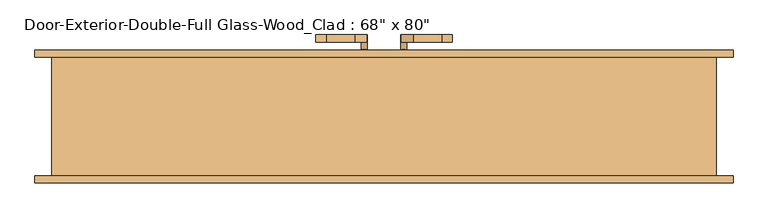
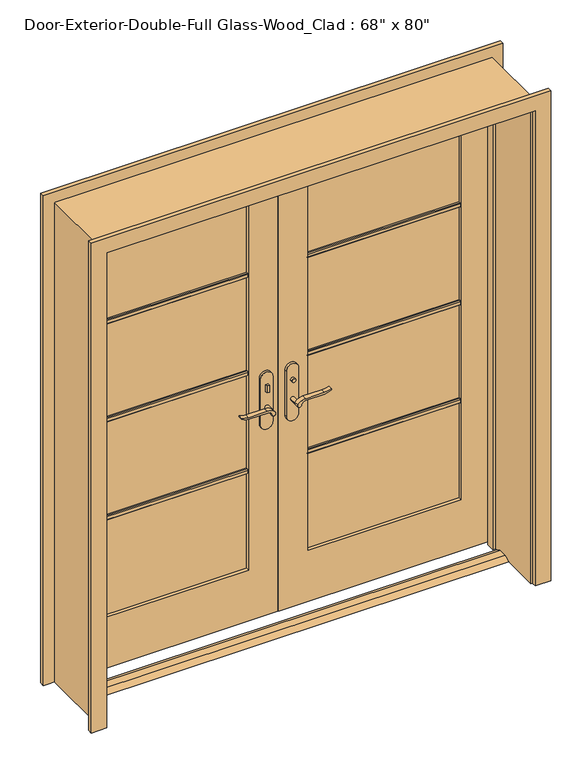
"""IFC4 building model written with IfcOpenShell, lengths in millimetres: door geometry."""

import ifcopenshell
import ifcopenshell.guid

model = None  # the IFC model being written
_history = None  # IfcOwnerHistory: only IFC2X3 demands one
_inside = {}  # id of a spatial element -> (the spatial element, [elements in it])
_under = {}  # id of a project, library or spatial element -> (it, [spatial elements below it])
_declared = {}  # id of a project -> (the project, [libraries it declares])
_typed = {}  # id of a type object -> (the type object, [elements of that type])
_made_of = {}  # id of a material, layer set ... -> (it, [elements and type objects made of it])


def new_model(schema):
    """Start an empty IFC model of exactly this schema.

    Asked for "IFC4X3", IfcOpenShell would pick the latest addendum, in which some entities
    have other attributes; the version numbers below select the first issue.
    IFC2X3 requires an IfcOwnerHistory on every rooted entity: one is made here for all.
    """
    global model, _history
    if schema == "IFC4X3":
        model = ifcopenshell.file(schema_version=(4, 3, 0, 0))
    else:
        model = ifcopenshell.file(schema=schema)
    _inside.clear()
    _under.clear()
    _declared.clear()
    _typed.clear()
    _made_of.clear()
    _history = None
    if model.schema == "IFC2X3":
        org = make("IfcOrganization", Name="unknown")
        user = make(
            "IfcPersonAndOrganization",
            ThePerson=make("IfcPerson", FamilyName="unknown"),
            TheOrganization=org,
        )
        app = make(
            "IfcApplication",
            ApplicationDeveloper=org,
            Version="unknown",
            ApplicationFullName="unknown",
            ApplicationIdentifier="unknown",
        )
        _history = make(
            "IfcOwnerHistory",
            OwningUser=user,
            OwningApplication=app,
            ChangeAction="ADDED",
            CreationDate=0,
        )
    return model


def make(cls, **values):
    """One entity of the class cls with the attributes given. An attribute that is None is left unset."""
    return model.create_entity(
        cls, **{name: value for name, value in values.items() if value is not None}
    )


def rooted(cls, **values):
    """An entity with a GlobalId (a new one), such as an element, a storey or a relation."""
    return make(cls, GlobalId=ifcopenshell.guid.new(), OwnerHistory=_history, **values)


def si_unit(unit_type, name, prefix=None):
    """IfcSIUnit, for example si_unit("LENGTHUNIT", "METRE", prefix="MILLI")."""
    return make("IfcSIUnit", UnitType=unit_type, Prefix=prefix, Name=name)


def assignment(units):
    """IfcUnitAssignment: the units of a project."""
    return None if units is None else make("IfcUnitAssignment", Units=units)


def point(xyz):
    """IfcCartesianPoint."""
    return None if xyz is None else make("IfcCartesianPoint", Coordinates=xyz)


def direction(xyz):
    """IfcDirection."""
    return None if xyz is None else make("IfcDirection", DirectionRatios=xyz)


def frame(location, z_axis=None, x_axis=None):
    """IfcAxis2Placement3D, a coordinate frame: its origin and axes. An axis left out is left unset."""
    return make(
        "IfcAxis2Placement3D",
        Location=point(location),
        Axis=direction(z_axis),
        RefDirection=direction(x_axis),
    )


def frame_2d(location, x_axis=None):
    """IfcAxis2Placement2D, a coordinate frame in the plane: its origin and x axis."""
    return make(
        "IfcAxis2Placement2D", Location=point(location), RefDirection=direction(x_axis)
    )


def origin():
    """The frame at (0, 0, 0) with its axes left unset."""
    return frame((0.0, 0.0, 0.0))


def place(relative_to, where):
    """IfcLocalPlacement: puts the frame where relative to a parent placement (None: the world)."""
    return make(
        "IfcLocalPlacement", PlacementRelTo=relative_to, RelativePlacement=where
    )


def context(
    kind, dimensions, precision=None, world=None, true_north=None, identifier=None
):
    """IfcGeometricRepresentationContext, for example the 3D "Model" context."""
    return make(
        "IfcGeometricRepresentationContext",
        ContextIdentifier=identifier,
        ContextType=kind,
        CoordinateSpaceDimension=dimensions,
        Precision=precision,
        WorldCoordinateSystem=world,
        TrueNorth=true_north,
    )


def project(units=None, contexts=None):
    """IfcProject with its units and contexts."""
    return rooted(
        "IfcProject",
        Name="project",
        RepresentationContexts=contexts,
        UnitsInContext=assignment(units),
    )


def spatial(cls, under=None, at=None, **own):
    """A site, building, storey or space (cls), placed at a placement, below another one or the project."""
    s = rooted(cls, ObjectPlacement=at, **own)
    if under is not None:
        _under.setdefault(under.id(), (under, []))[1].append(s)
    return s


def polyline(points):
    """IfcPolyline through the points."""
    return make("IfcPolyline", Points=[point(p) for p in points])


def circle_curve(where, radius):
    """IfcCircle in the frame where."""
    return make("IfcCircle", Position=where, Radius=radius)


def trimmed(basis, trim1, trim2, sense, master):
    """IfcTrimmedCurve: the piece of a basis curve between two trims."""
    return make(
        "IfcTrimmedCurve",
        BasisCurve=basis,
        Trim1=trim1,
        Trim2=trim2,
        SenseAgreement=sense,
        MasterRepresentation=master,
    )


def segment(curve, same_sense, transition):
    """IfcCompositeCurveSegment."""
    return make(
        "IfcCompositeCurveSegment",
        Transition=transition,
        SameSense=same_sense,
        ParentCurve=curve,
    )


def composite_curve(segments, self_intersect=None):
    """IfcCompositeCurve: segments joined end to end."""
    return make("IfcCompositeCurve", Segments=segments, SelfIntersect=self_intersect)


def outline(outer, holes=None, kind="AREA"):
    """IfcArbitraryClosedProfileDef: a profile drawn as a closed curve; with holes, ...WithVoids."""
    if holes is None:
        return make("IfcArbitraryClosedProfileDef", ProfileType=kind, OuterCurve=outer)
    return make(
        "IfcArbitraryProfileDefWithVoids",
        ProfileType=kind,
        OuterCurve=outer,
        InnerCurves=holes,
    )


def extrude(swept, where, along, depth):
    """IfcExtrudedAreaSolid: the profile swept, set in the frame where, extruded along a direction by depth."""
    return make(
        "IfcExtrudedAreaSolid",
        SweptArea=swept,
        Position=where,
        ExtrudedDirection=direction(along),
        Depth=depth,
    )


def faces_of(points, faces, orient=None, outer=None):
    """IfcFace entities. A face is a list of loops; a loop is a list of indices into points, from 0.

    orient and outer hold one flag for each loop. By default every Orientation is true, the
    first loop of a face is its IfcFaceOuterBound and the others are IfcFaceBound.
    """
    made = []
    for i, loops in enumerate(faces):
        bounds = []
        for j, loop in enumerate(loops):
            is_outer = j == 0 if outer is None else outer[i][j]
            bounds.append(
                make(
                    "IfcFaceOuterBound" if is_outer else "IfcFaceBound",
                    Bound=make("IfcPolyLoop", Polygon=[points[k] for k in loop]),
                    Orientation=True if orient is None else orient[i][j],
                )
            )
        made.append(make("IfcFace", Bounds=bounds))
    return made


def faceted_brep(points, faces, orient=None, outer=None, voids=None):
    """IfcFacetedBrep: a solid bounded by flat faces; with voids (closed shells), ...WithVoids."""
    shared = [point(p) for p in points]
    hull = make("IfcClosedShell", CfsFaces=faces_of(shared, faces, orient, outer))
    if voids is None:
        return make("IfcFacetedBrep", Outer=hull)
    return make(
        "IfcFacetedBrepWithVoids",
        Outer=hull,
        Voids=[
            make(cls, CfsFaces=faces_of(shared, fs, o, b)) for cls, fs, o, b in voids
        ],
    )


def shape(context_of_items, identifier, shape_type, items):
    """IfcShapeRepresentation: the items that make up one representation, for example the "Body"."""
    return make(
        "IfcShapeRepresentation",
        ContextOfItems=context_of_items,
        RepresentationIdentifier=identifier,
        RepresentationType=shape_type,
        Items=items,
    )


def source(mapping_origin, context_of_items, identifier, shape_type, items):
    """IfcRepresentationMap: a shape defined once, which mapped items show again and again."""
    return make(
        "IfcRepresentationMap",
        MappingOrigin=mapping_origin,
        MappedRepresentation=shape(context_of_items, identifier, shape_type, items),
    )


def transform(
    local_origin,
    x_axis=None,
    y_axis=None,
    z_axis=None,
    scale=None,
    scale2=None,
    scale3=None,
    uniform=True,
):
    """IfcCartesianTransformationOperator3D, or its non-uniform kind. x_axis, y_axis, z_axis: its Axis1, 2, 3."""
    if uniform:
        return make(
            "IfcCartesianTransformationOperator3D",
            Axis1=direction(x_axis),
            Axis2=direction(y_axis),
            LocalOrigin=point(local_origin),
            Scale=scale,
            Axis3=direction(z_axis),
        )
    return make(
        "IfcCartesianTransformationOperator3DnonUniform",
        Axis1=direction(x_axis),
        Axis2=direction(y_axis),
        LocalOrigin=point(local_origin),
        Scale=scale,
        Axis3=direction(z_axis),
        Scale2=scale2,
        Scale3=scale3,
    )


def mapped(mapping_source, mapping_target):
    """IfcMappedItem: shows the shape of a source again, moved by a transform."""
    return make(
        "IfcMappedItem", MappingSource=mapping_source, MappingTarget=mapping_target
    )


def made_of(thing, what):
    """Note that an element or type object is made of a material, layer set ...; save() writes the relation."""
    if what is not None:
        _made_of.setdefault(what.id(), (what, []))[1].append(thing)
    return thing


def element(
    cls,
    number,
    at=None,
    inside=None,
    cuts=None,
    type_object=None,
    material=None,
    context=None,
    identifier="Body",
    shape_type=None,
    held_by="IfcProductDefinitionShape",
    body=None,
    shapes=None,
    **own,
):
    """One element of the class cls, such as IfcWall. Its Tag is "e" and its number.

    at: its placement. inside: the storey or other place that contains it. cuts: it is an
    opening in that element (IfcRelVoidsElement). A single representation is given by context,
    identifier, shape_type and body (its items); several are given by shapes. held_by: the class
    of the entity that holds the representations. save() writes the other relations.
    """
    e = rooted(cls, Tag="e%d" % number, ObjectPlacement=at, **own)
    if body is not None:
        shapes = [shape(context, identifier, shape_type, body)]
    if shapes is not None:
        e.Representation = make(held_by, Representations=shapes)
    if inside is not None:
        _inside.setdefault(inside.id(), (inside, []))[1].append(e)
    if cuts is not None:
        rooted(
            "IfcRelVoidsElement", RelatingBuildingElement=cuts, RelatedOpeningElement=e
        )
    if type_object is not None:
        _typed.setdefault(type_object.id(), (type_object, []))[1].append(e)
    return made_of(e, material)


def aggregate(whole, parts):
    """IfcRelAggregates: a whole, such as a stair, and the parts it consists of."""
    return rooted("IfcRelAggregates", RelatingObject=whole, RelatedObjects=parts)


def save(model, path):
    """Write the relations noted so far, then the file.

    IfcRelAggregates (storeys below a building ...), IfcRelContainedInSpatialStructure (elements
    in a storey), IfcRelDefinesByType, IfcRelAssociatesMaterial and IfcRelDeclares: one each for
    every whole, place, type object, material and project.
    """
    for whole, parts in _under.values():
        aggregate(whole, parts)
    for where, things in _inside.values():
        rooted(
            "IfcRelContainedInSpatialStructure",
            RelatedElements=things,
            RelatingStructure=where,
        )
    for kind, things in _typed.values():
        rooted("IfcRelDefinesByType", RelatedObjects=things, RelatingType=kind)
    for what, things in _made_of.values():
        rooted("IfcRelAssociatesMaterial", RelatedObjects=things, RelatingMaterial=what)
    for by, libraries in _declared.values():
        rooted("IfcRelDeclares", RelatingContext=by, RelatedDefinitions=libraries)
    model.write(path)


def door_97aac55e(model_context):
    return source(origin(), model_context, "Body", "SolidModel", [
        extrude(outline(polyline([(19.05, 12.7), (53.975, 12.7), (79.375, 0.0), (-6.35, 0.0), (19.05, 12.7)])), frame((-863.6, 0.0, 0.0), z_axis=(1.0, 0.0, 0.0), x_axis=(0.0, 1.0, 0.0)), (0.0, 0.0, 1.0), 1727.2),
        extrude(outline(polyline([(-47.4019111, 100.65), (-57.4019111, 100.65), (-57.4019111, 110.65), (-47.4019111, 110.65), (-47.4019111, 100.65)])), frame((0.0, 0.0, 981.9), z_axis=(0.0, 0.0, 1.0), x_axis=(1.0, 0.0, 0.0)), (0.0, 0.0, 1.0), 30.0),
        extrude(outline(composite_curve([segment(trimmed(circle_curve(frame_2d((996.9, -52.4019111)), 8.0), [point((996.9, -60.4019111))], [point((996.9, -44.4019111))], False, "CARTESIAN"), True, "CONTINUOUS"), segment(trimmed(circle_curve(frame_2d((996.9, -52.4019111)), 8.0), [point((996.9, -44.4019111))], [point((996.9, -60.4019111))], False, "CARTESIAN"), True, "CONTINUOUS")], self_intersect=False)), frame((0.0, 165.575, 0.0), z_axis=(0.0, 1.0, 0.0), x_axis=(0.0, 0.0, 1.0)), (0.0, 0.0, 1.0), 10.0),
        extrude(outline(composite_curve([segment(trimmed(circle_curve(frame_2d((897.1555521, -76.0694241)), 37.2832219), [point((919.0523287, -45.8937749))], [point((934.4, -77.7693445))], False, "CARTESIAN"), True, "CONTINUOUS"), segment(polyline([(934.4, -77.7693445), (934.4, -154.045502)]), True, "CONTINUOUS"), segment(trimmed(circle_curve(frame_2d((1017.6850638, -153.9791202)), 83.2850902), [point((934.4, -154.045502))], [point((939.4, -182.4019111))], True, "CARTESIAN"), True, "CONTINUOUS"), segment(polyline([(939.4, -182.4019111), (936.6135558, -182.4019111)]), True, "CONTINUOUS"), segment(trimmed(circle_curve(frame_2d((986.6709207, -150.4622499)), 59.3791355), [point((936.6135558, -182.4019111))], [point((927.4, -154.045502))], False, "CARTESIAN"), True, "CONTINUOUS"), segment(polyline([(927.4, -154.045502), (927.4, -77.7881013)]), True, "CONTINUOUS"), segment(trimmed(circle_curve(frame_2d((909.2738613, -77.7881013)), 18.1261387), [point((927.4, -77.7881013))], [point((914.4, -60.4019111))], True, "CARTESIAN"), True, "CONTINUOUS"), segment(trimmed(circle_curve(frame_2d((914.4, -52.4019111)), 8.0), [point((914.4, -60.4019111))], [point((919.0523287, -45.8937749))], False, "CARTESIAN"), True, "CONTINUOUS")], self_intersect=False)), frame((0.0, 60.65, 0.0), z_axis=(0.0, 1.0, 0.0), x_axis=(0.0, 0.0, 1.0)), (0.0, 0.0, 1.0), 20.0),
        extrude(outline(composite_curve([segment(trimmed(circle_curve(frame_2d((914.4, -52.4019111)), 8.0), [point((914.3999903, -60.4019111))], [point((919.0523287, -45.8937749))], False, "CARTESIAN"), True, "CONTINUOUS"), segment(trimmed(circle_curve(frame_2d((897.1555521, -76.0694241)), 37.2832219), [point((919.0523287, -45.8937749))], [point((934.4, -77.7693445))], False, "CARTESIAN"), True, "CONTINUOUS"), segment(polyline([(934.4, -77.7693445), (934.4, -154.045502)]), True, "CONTINUOUS"), segment(trimmed(circle_curve(frame_2d((1017.6850638, -153.9791202)), 83.2850902), [point((934.4, -154.045502))], [point((939.4, -182.4019111))], True, "CARTESIAN"), True, "CONTINUOUS"), segment(polyline([(939.4, -182.4019111), (936.6135558, -182.4019111)]), True, "CONTINUOUS"), segment(trimmed(circle_curve(frame_2d((986.6709207, -150.4622499)), 59.3791355), [point((936.6135558, -182.4019111))], [point((927.4, -154.045502))], False, "CARTESIAN"), True, "CONTINUOUS"), segment(polyline([(927.4, -154.045502), (927.4, -77.788099)]), True, "CONTINUOUS"), segment(trimmed(circle_curve(frame_2d((909.2738682, -77.788099)), 18.1261318), [point((927.4, -77.788099))], [point((914.3999903, -60.4019111))], True, "CARTESIAN"), True, "CONTINUOUS")], self_intersect=False)), frame((0.0, 195.575, 0.0), z_axis=(0.0, 1.0, 0.0), x_axis=(0.0, 0.0, 1.0)), (0.0, 0.0, 1.0), 20.0),
        extrude(outline(composite_curve([segment(trimmed(circle_curve(frame_2d((914.4, -52.4019111)), 8.0), [point((914.4, -60.4019111))], [point((914.4, -44.4019111))], False, "CARTESIAN"), True, "CONTINUOUS"), segment(trimmed(circle_curve(frame_2d((914.4, -52.4019111)), 8.0), [point((914.4, -44.4019111))], [point((914.4, -60.4019111))], False, "CARTESIAN"), True, "CONTINUOUS")], self_intersect=False)), frame((0.0, 80.65, 0.0), z_axis=(0.0, 1.0, 0.0), x_axis=(0.0, 0.0, 1.0)), (0.0, 0.0, 1.0), 30.0),
        extrude(outline(composite_curve([segment(trimmed(circle_curve(frame_2d((914.4, -52.4019111)), 8.0), [point((914.4, -60.4019111))], [point((914.4, -44.4019111))], False, "CARTESIAN"), True, "CONTINUOUS"), segment(trimmed(circle_curve(frame_2d((914.4, -52.4019111)), 8.0), [point((914.4, -44.4019111))], [point((914.4, -60.4019111))], False, "CARTESIAN"), True, "CONTINUOUS")], self_intersect=False)), frame((0.0, 165.575, 0.0), z_axis=(0.0, 1.0, 0.0), x_axis=(0.0, 0.0, 1.0)), (0.0, 0.0, 1.0), 30.0),
        extrude(outline(composite_curve([segment(polyline([(844.4, -27.4019111), (1039.4, -27.4019111)]), True, "CONTINUOUS"), segment(trimmed(circle_curve(frame_2d((1039.4, -52.4019111)), 25.0), [point((1039.4, -27.4019111))], [point((1039.4, -77.4019111))], False, "CARTESIAN"), True, "CONTINUOUS"), segment(polyline([(1039.4, -77.4019111), (844.4, -77.4019111)]), True, "CONTINUOUS"), segment(trimmed(circle_curve(frame_2d((844.4, -52.4019111)), 25.0), [point((844.4, -77.4019111))], [point((844.4, -27.4019111))], False, "CARTESIAN"), True, "CONTINUOUS")], self_intersect=False)), frame((0.0, 110.65, 0.0), z_axis=(0.0, 1.0, 0.0), x_axis=(0.0, 0.0, 1.0)), (0.0, 0.0, 1.0), 10.0),
        extrude(outline(composite_curve([segment(polyline([(844.4, -27.4019111), (1039.4, -27.4019111)]), True, "CONTINUOUS"), segment(trimmed(circle_curve(frame_2d((1039.4, -52.4019111)), 25.0), [point((1039.4, -27.4019111))], [point((1039.4, -77.4019111))], False, "CARTESIAN"), True, "CONTINUOUS"), segment(polyline([(1039.4, -77.4019111), (844.4, -77.4019111)]), True, "CONTINUOUS"), segment(trimmed(circle_curve(frame_2d((844.4, -52.4019111)), 25.0), [point((844.4, -77.4019111))], [point((844.4, -27.4019111))], False, "CARTESIAN"), True, "CONTINUOUS")], self_intersect=False)), frame((0.0, 155.575, 0.0), z_axis=(0.0, 1.0, 0.0), x_axis=(0.0, 0.0, 1.0)), (0.0, 0.0, 1.0), 10.0),
        extrude(outline(polyline([(47.3875, 175.575), (57.3875, 175.575), (57.3875, 165.575), (47.3875, 165.575), (47.3875, 175.575)])), frame((0.0, 0.0, 981.9), z_axis=(0.0, 0.0, 1.0), x_axis=(1.0, 0.0, 0.0)), (0.0, 0.0, 1.0), 30.0),
        extrude(outline(composite_curve([segment(trimmed(circle_curve(frame_2d((996.9, 52.3875)), 8.0), [point((996.9, 60.3875))], [point((996.9, 44.3875))], False, "CARTESIAN"), True, "CONTINUOUS"), segment(trimmed(circle_curve(frame_2d((996.9, 52.3875)), 8.0), [point((996.9, 44.3875))], [point((996.9, 60.3875))], False, "CARTESIAN"), True, "CONTINUOUS")], self_intersect=False)), frame((0.0, 100.65, 0.0), z_axis=(0.0, 1.0, 0.0), x_axis=(0.0, 0.0, 1.0)), (0.0, 0.0, 1.0), 10.0),
        extrude(outline(composite_curve([segment(trimmed(circle_curve(frame_2d((914.4, 52.3875)), 8.0), [point((919.0523287, 45.8793637))], [point((914.4, 60.3875))], False, "CARTESIAN"), True, "CONTINUOUS"), segment(trimmed(circle_curve(frame_2d((909.2738613, 77.7736901)), 18.1261387), [point((914.4, 60.3875))], [point((927.4, 77.7736901))], True, "CARTESIAN"), True, "CONTINUOUS"), segment(polyline([(927.4, 77.7736901), (927.4, 154.0310909)]), True, "CONTINUOUS"), segment(trimmed(circle_curve(frame_2d((986.6709207, 150.4478388)), 59.3791355), [point((927.4, 154.0310909))], [point((936.6135558, 182.3875))], False, "CARTESIAN"), True, "CONTINUOUS"), segment(polyline([(936.6135558, 182.3875), (939.4, 182.3875)]), True, "CONTINUOUS"), segment(trimmed(circle_curve(frame_2d((1017.6850638, 153.9647091)), 83.2850902), [point((939.4, 182.3875))], [point((934.4, 154.0310909))], True, "CARTESIAN"), True, "CONTINUOUS"), segment(polyline([(934.4, 154.0310909), (934.4, 77.7549333)]), True, "CONTINUOUS"), segment(trimmed(circle_curve(frame_2d((897.1555521, 76.0550129)), 37.2832219), [point((934.4, 77.7549333))], [point((919.0523287, 45.8793637))], False, "CARTESIAN"), True, "CONTINUOUS")], self_intersect=False)), frame((0.0, 195.575, 0.0), z_axis=(0.0, 1.0, 0.0), x_axis=(0.0, 0.0, 1.0)), (0.0, 0.0, 1.0), 20.0),
        extrude(outline(composite_curve([segment(trimmed(circle_curve(frame_2d((909.2738682, 77.7736878)), 18.1261318), [point((914.3999903, 60.3875))], [point((927.4, 77.7736878))], True, "CARTESIAN"), True, "CONTINUOUS"), segment(polyline([(927.4, 77.7736878), (927.4, 154.0310909)]), True, "CONTINUOUS"), segment(trimmed(circle_curve(frame_2d((986.6709207, 150.4478388)), 59.3791355), [point((927.4, 154.0310909))], [point((936.6135558, 182.3875))], False, "CARTESIAN"), True, "CONTINUOUS"), segment(polyline([(936.6135558, 182.3875), (939.4, 182.3875)]), True, "CONTINUOUS"), segment(trimmed(circle_curve(frame_2d((1017.6850638, 153.9647091)), 83.2850902), [point((939.4, 182.3875))], [point((934.4, 154.0310909))], True, "CARTESIAN"), True, "CONTINUOUS"), segment(polyline([(934.4, 154.0310909), (934.4, 77.7549333)]), True, "CONTINUOUS"), segment(trimmed(circle_curve(frame_2d((897.1555521, 76.0550129)), 37.2832219), [point((934.4, 77.7549333))], [point((919.0523287, 45.8793637))], False, "CARTESIAN"), True, "CONTINUOUS"), segment(trimmed(circle_curve(frame_2d((914.4, 52.3875)), 8.0), [point((919.0523287, 45.8793637))], [point((914.3999903, 60.3875))], False, "CARTESIAN"), True, "CONTINUOUS")], self_intersect=False)), frame((0.0, 60.65, 0.0), z_axis=(0.0, 1.0, 0.0), x_axis=(0.0, 0.0, 1.0)), (0.0, 0.0, 1.0), 20.0),
        extrude(outline(composite_curve([segment(trimmed(circle_curve(frame_2d((914.4, 52.3875)), 8.0), [point((914.4, 60.3875))], [point((914.4, 44.3875))], False, "CARTESIAN"), True, "CONTINUOUS"), segment(trimmed(circle_curve(frame_2d((914.4, 52.3875)), 8.0), [point((914.4, 44.3875))], [point((914.4, 60.3875))], False, "CARTESIAN"), True, "CONTINUOUS")], self_intersect=False)), frame((0.0, 165.575, 0.0), z_axis=(0.0, 1.0, 0.0), x_axis=(0.0, 0.0, 1.0)), (0.0, 0.0, 1.0), 30.0),
        extrude(outline(composite_curve([segment(trimmed(circle_curve(frame_2d((914.4, 52.3875)), 8.0), [point((914.4, 60.3875))], [point((914.4, 44.3875))], False, "CARTESIAN"), True, "CONTINUOUS"), segment(trimmed(circle_curve(frame_2d((914.4, 52.3875)), 8.0), [point((914.4, 44.3875))], [point((914.4, 60.3875))], False, "CARTESIAN"), True, "CONTINUOUS")], self_intersect=False)), frame((0.0, 80.65, 0.0), z_axis=(0.0, 1.0, 0.0), x_axis=(0.0, 0.0, 1.0)), (0.0, 0.0, 1.0), 30.0),
        extrude(outline(composite_curve([segment(trimmed(circle_curve(frame_2d((844.4, 52.3875)), 25.0), [point((844.4, 27.3875))], [point((844.4, 77.3875))], False, "CARTESIAN"), True, "CONTINUOUS"), segment(polyline([(844.4, 77.3875), (1039.4, 77.3875)]), True, "CONTINUOUS"), segment(trimmed(circle_curve(frame_2d((1039.4, 52.3875)), 25.0), [point((1039.4, 77.3875))], [point((1039.4, 27.3875))], False, "CARTESIAN"), True, "CONTINUOUS"), segment(polyline([(1039.4, 27.3875), (844.4, 27.3875)]), True, "CONTINUOUS")], self_intersect=False)), frame((0.0, 155.575, 0.0), z_axis=(0.0, 1.0, 0.0), x_axis=(0.0, 0.0, 1.0)), (0.0, 0.0, 1.0), 10.0),
        extrude(outline(composite_curve([segment(trimmed(circle_curve(frame_2d((844.4, 52.3875)), 25.0), [point((844.4, 27.3875))], [point((844.4, 77.3875))], False, "CARTESIAN"), True, "CONTINUOUS"), segment(polyline([(844.4, 77.3875), (1039.4, 77.3875)]), True, "CONTINUOUS"), segment(trimmed(circle_curve(frame_2d((1039.4, 52.3875)), 25.0), [point((1039.4, 77.3875))], [point((1039.4, 27.3875))], False, "CARTESIAN"), True, "CONTINUOUS"), segment(polyline([(1039.4, 27.3875), (844.4, 27.3875)]), True, "CONTINUOUS")], self_intersect=False)), frame((0.0, 110.65, 0.0), z_axis=(0.0, 1.0, 0.0), x_axis=(0.0, 0.0, 1.0)), (0.0, 0.0, 1.0), 10.0),
        extrude(outline(polyline([(134.62, 1502.171875), (134.62, 1483.121875), (128.27, 1483.121875), (125.095, 1486.296875), (125.095, 1498.996875), (128.27, 1502.171875), (134.62, 1502.171875)])), frame((120.65, 0.0, 0.0), z_axis=(1.0, 0.0, 0.0), x_axis=(0.0, 1.0, 0.0)), (0.0, 0.0, 1.0), 622.3),
        extrude(outline(polyline([(134.62, 1081.88125), (134.62, 1062.83125), (128.27, 1062.83125), (125.095, 1066.00625), (125.095, 1078.70625), (128.27, 1081.88125), (134.62, 1081.88125)])), frame((120.65, 0.0, 0.0), z_axis=(1.0, 0.0, 0.0), x_axis=(0.0, 1.0, 0.0)), (0.0, 0.0, 1.0), 622.3),
        extrude(outline(polyline([(134.62, 661.590625), (134.62, 642.540625), (128.27, 642.540625), (125.095, 645.715625), (125.095, 658.415625), (128.27, 661.590625), (134.62, 661.590625)])), frame((120.65, 0.0, 0.0), z_axis=(1.0, 0.0, 0.0), x_axis=(0.0, 1.0, 0.0)), (0.0, 0.0, 1.0), 622.3),
        extrude(outline(polyline([(141.605, 1502.171875), (147.955, 1502.171875), (151.13, 1498.996875), (151.13, 1486.296875), (147.955, 1483.121875), (141.605, 1483.121875), (141.605, 1502.171875)])), frame((-742.95, 0.0, 0.0), z_axis=(1.0, 0.0, 0.0), x_axis=(0.0, 1.0, 0.0)), (0.0, 0.0, 1.0), 622.3),
        extrude(outline(polyline([(141.605, 1081.88125), (147.955, 1081.88125), (151.13, 1078.70625), (151.13, 1066.00625), (147.955, 1062.83125), (141.605, 1062.83125), (141.605, 1081.88125)])), frame((-742.95, 0.0, 0.0), z_axis=(1.0, 0.0, 0.0), x_axis=(0.0, 1.0, 0.0)), (0.0, 0.0, 1.0), 622.3),
        extrude(outline(polyline([(141.605, 661.590625), (147.955, 661.590625), (151.13, 658.415625), (151.13, 645.715625), (147.955, 642.540625), (141.605, 642.540625), (141.605, 661.590625)])), frame((-742.95, 0.0, 0.0), z_axis=(1.0, 0.0, 0.0), x_axis=(0.0, 1.0, 0.0)), (0.0, 0.0, 1.0), 622.3),
        extrude(outline(polyline([(141.605, 1502.171875), (147.955, 1502.171875), (151.13, 1498.996875), (151.13, 1486.296875), (147.955, 1483.121875), (141.605, 1483.121875), (141.605, 1502.171875)])), frame((120.65, 0.0, 0.0), z_axis=(1.0, 0.0, 0.0), x_axis=(0.0, 1.0, 0.0)), (0.0, 0.0, 1.0), 622.3),
        extrude(outline(polyline([(141.605, 1081.88125), (147.955, 1081.88125), (151.13, 1078.70625), (151.13, 1066.00625), (147.955, 1062.83125), (141.605, 1062.83125), (141.605, 1081.88125)])), frame((120.65, 0.0, 0.0), z_axis=(1.0, 0.0, 0.0), x_axis=(0.0, 1.0, 0.0)), (0.0, 0.0, 1.0), 622.3),
        extrude(outline(polyline([(141.605, 661.590625), (147.955, 661.590625), (151.13, 658.415625), (151.13, 645.715625), (147.955, 642.540625), (141.605, 642.540625), (141.605, 661.590625)])), frame((120.65, 0.0, 0.0), z_axis=(1.0, 0.0, 0.0), x_axis=(0.0, 1.0, 0.0)), (0.0, 0.0, 1.0), 622.3),
        extrude(outline(polyline([(134.62, 1502.171875), (134.62, 1483.121875), (128.27, 1483.121875), (125.095, 1486.296875), (125.095, 1498.996875), (128.27, 1502.171875), (134.62, 1502.171875)])), frame((-742.95, 0.0, 0.0), z_axis=(1.0, 0.0, 0.0), x_axis=(0.0, 1.0, 0.0)), (0.0, 0.0, 1.0), 622.3),
        extrude(outline(polyline([(134.62, 1081.88125), (134.62, 1062.83125), (128.27, 1062.83125), (125.095, 1066.00625), (125.095, 1078.70625), (128.27, 1081.88125), (134.62, 1081.88125)])), frame((-742.95, 0.0, 0.0), z_axis=(1.0, 0.0, 0.0), x_axis=(0.0, 1.0, 0.0)), (0.0, 0.0, 1.0), 622.3),
        extrude(outline(polyline([(134.62, 661.590625), (134.62, 642.540625), (128.27, 642.540625), (125.095, 645.715625), (125.095, 658.415625), (128.27, 661.590625), (134.62, 661.590625)])), frame((-742.95, 0.0, 0.0), z_axis=(1.0, 0.0, 0.0), x_axis=(0.0, 1.0, 0.0)), (0.0, 0.0, 1.0), 622.3),
        extrude(outline(polyline([(0.0, 869.95), (0.0, 933.45), (2101.85, 933.45), (2101.85, -933.45), (0.0, -933.45), (0.0, -869.95), (2038.35, -869.95), (2038.35, 869.95), (0.0, 869.95)])), frame((0.0, 155.575, 0.0), z_axis=(0.0, 1.0, 0.0), x_axis=(0.0, 0.0, 1.0)), (0.0, 0.0, 1.0), 19.05),
        extrude(outline(polyline([(0.0, 869.95), (0.0, 933.45), (2101.85, 933.45), (2101.85, -933.45), (0.0, -933.45), (0.0, -869.95), (2038.35, -869.95), (2038.35, 869.95), (0.0, 869.95)])), frame((0.0, -180.975, 0.0), z_axis=(0.0, 1.0, 0.0), x_axis=(0.0, 0.0, 1.0)), (0.0, 0.0, 1.0), 19.05),
        extrude(outline(polyline([(12.7, 863.6), (2032.0, 863.6), (2032.0, 1.5875), (12.7, 1.5875), (12.7, 863.6)]), holes=[polyline([(1912.9375, 120.65), (1912.9375, 742.95), (231.775, 742.95), (231.775, 120.65), (1912.9375, 120.65)])]), frame((0.0, 120.65, 0.0), z_axis=(0.0, 1.0, 0.0), x_axis=(0.0, 0.0, 1.0)), (0.0, 0.0, 1.0), 34.925),
        extrude(outline(polyline([(2032.0, -863.6), (12.7, -863.6), (12.7, -1.6019111), (2032.0, -1.6019111), (2032.0, -863.6)]), holes=[polyline([(231.775, -742.95), (1912.9375, -742.95), (1912.9375, -120.65), (231.775, -120.65), (231.775, -742.95)])]), frame((0.0, 120.65, 0.0), z_axis=(0.0, 1.0, 0.0), x_axis=(0.0, 0.0, 1.0)), (0.0, 0.0, 1.0), 34.925),
        faceted_brep([(889.0, 155.575, 0.0), (889.0, -161.925, 0.0), (863.6, -161.925, 0.0), (863.6, 85.725, 0.0), (850.9, 85.725, 0.0), (850.9, 120.65, 0.0), (863.6, 120.65, 0.0), (863.6, 155.575, 0.0), (889.0, 155.575, 2057.4), (889.0, -161.925, 2057.4), (-889.0, -161.925, 2057.4), (-889.0, -161.925, 0.0), (-863.6, -161.925, 0.0), (-863.6, -161.925, 2032.0), (863.6, -161.925, 2032.0), (863.6, 85.725, 2032.0), (-863.6, 85.725, 2032.0), (-863.6, 85.725, 0.0), (-850.9, 85.725, 0.0), (-850.9, 85.725, 2019.3), (850.9, 85.725, 2019.3), (850.9, 120.65, 2019.3), (1.5875, 120.65, 2019.3), (-1.6019111, 120.65, 2019.3), (-850.9, 120.65, 2019.3), (-850.9, 120.65, 0.0), (-863.6, 120.65, 0.0), (-863.6, 120.65, 2032.0), (-1.6019111, 120.65, 2032.0), (1.5875, 120.65, 2032.0), (863.6, 120.65, 2032.0), (863.6, 155.575, 2032.0), (1.5875, 155.575, 2032.0), (-1.6019111, 155.575, 2032.0), (-863.6, 155.575, 2032.0), (-863.6, 155.575, 0.0), (-889.0, 155.575, 0.0), (-889.0, 155.575, 2057.4)], [[[0, 1, 2, 3, 4, 5, 6, 7]], [[1, 0, 8, 9]], [[2, 1, 9, 10, 11, 12, 13, 14]], [[3, 2, 14, 15]], [[4, 3, 15, 16, 17, 18, 19, 20]], [[5, 4, 20, 21]], [[6, 5, 21, 22, 23, 24, 25, 26, 27, 28, 29, 30]], [[7, 6, 30, 31]], [[0, 7, 31, 32, 33, 34, 35, 36, 37, 8]], [[9, 8, 37, 10]], [[14, 13, 16, 15]], [[20, 19, 24, 23, 22, 21]], [[31, 30, 29, 28, 27, 34, 33, 32]], [[12, 11, 36, 35, 26, 25, 18, 17]], [[11, 10, 37, 36]], [[13, 12, 17, 16]], [[19, 18, 25, 24]], [[27, 26, 35, 34]]]),
        extrude(outline(polyline([(742.95, 134.62), (120.65, 134.62), (120.65, 141.605), (742.95, 141.605), (742.95, 134.62)])), frame((0.0, 0.0, 231.775), z_axis=(0.0, 0.0, 1.0), x_axis=(1.0, 0.0, 0.0)), (0.0, 0.0, 1.0), 1681.1625),
        extrude(outline(polyline([(-120.65, 134.62), (-742.95, 134.62), (-742.95, 141.605), (-120.65, 141.605), (-120.65, 134.62)])), frame((0.0, 0.0, 231.775), z_axis=(0.0, 0.0, 1.0), x_axis=(1.0, 0.0, 0.0)), (0.0, 0.0, 1.0), 1681.1625),
    ])


if __name__ == "__main__":
    model = new_model("IFC4")
    model_context = context("Model", 3, world=origin())
    ifc_project = project(units=[si_unit("LENGTHUNIT", "METRE", prefix="MILLI")], contexts=[model_context])
    site = spatial("IfcSite", under=ifc_project)
    building = spatial("IfcBuilding", under=site)
    placement = place(None, origin())
    door_shape = door_97aac55e(model_context)
    element("IfcDoor", 1, ObjectType="Door-Exterior-Double-Full Glass-Wood_Clad : 68\" x 80\"", at=placement, inside=building, context=model_context, shape_type="MappedRepresentation", body=[
        mapped(door_shape, transform((0.0, 0.0, 0.0), x_axis=(1.0, 0.0, 0.0), y_axis=(0.0, 1.0, 0.0), z_axis=(0.0, 0.0, 1.0))),
    ])
    save(model, "model.ifc")

# Revit data of these elements
# Type "Door-Exterior-Double-Full Glass-Wood_Clad : 68\" x 80\""
#   Type Mark = "21"
#   Assembly Code = "B2030100"
#   Analytic Construction = "French door, wood frame with double glass"
#   Top Rail = 0' - 4 11/16"
#   Threshold Offset [instance default] = 0' - 0 1/2"
#   Thickness = 0' - 1 3/8"
#   Thermal Resistance (R) = 1.9158 (h·ft²·°F)/BTU
#   Swing Angle [instance default] = 90.0000°
#   Stiles = 0' - 4 3/4"
#   Rough Width = 5' - 10"
#   Rough Height = 6' - 9"
#   Panel Width = 2' - 10"
#   Door Offset [instance default] = 0' - 0"
#   Height = 6' - 8"
#   Width = 5' - 8"
#   Heat Transfer Coefficient (U) = 0.5220 BTU/(h·ft²·°F)
#   Bottom Rail = 0' - 9 1/8"
#   Exterior Trim [instance default] = yes
#   Threshold [instance default] = yes
#   Show Grill [instance default] = yes
#   Function = 1
#   Trim Material = Cherry
#   Threshold Material = Cherry
#   Panel Material = Cherry
#   Glazing = Glass
#   Frame Material = Cherry
#   Door Handle Material = Aluminum
#   Visual Light Transmittance = 0
#   Solar Heat Gain Coefficient = 0
#   Wall Closure = (empty or 0)
#   Construction Type = (empty or 0)
# Element 1 (IfcDoor, "Door-Exterior-Double-Full Glass-Wood_Clad : 68\" x 80\"")
#   Materials on its faces: "Cherry", "Aluminum", "Glass"
# Materials
#   "Cherry": class "Wood", colour RGB 226 177 128, transparency 0, Description = "Prunus Serotina", Cost = 0
#   "Glass": class "Glass", colour RGB 0 128 192, transparency 0.75, Description = "Soda Lime Glass", Cost = 0
#   "Aluminum": class "Metal", colour RGB 247 247 247, transparency 0, Description = "Aluminum 6061", Cost = 0
